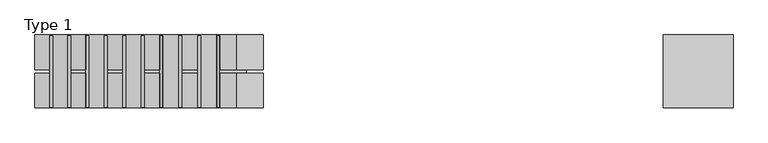
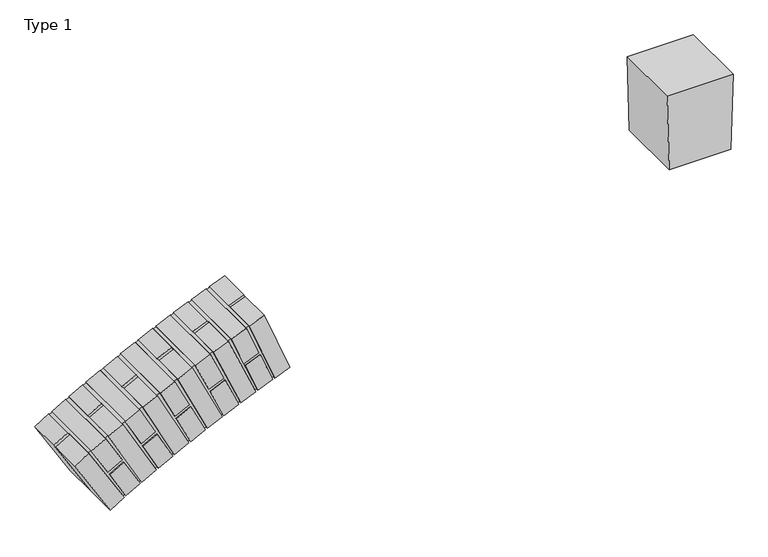
"""IFC4 building model written with IfcOpenShell, lengths in millimetres: proxy geometry, 00_GM_toog : Type 1."""

import ifcopenshell
import ifcopenshell.guid

model = None  # the IFC model being written
_history = None  # IfcOwnerHistory: only IFC2X3 demands one
_inside = {}  # id of a spatial element -> (the spatial element, [elements in it])
_under = {}  # id of a project, library or spatial element -> (it, [spatial elements below it])
_declared = {}  # id of a project -> (the project, [libraries it declares])
_typed = {}  # id of a type object -> (the type object, [elements of that type])
_made_of = {}  # id of a material, layer set ... -> (it, [elements and type objects made of it])


def new_model(schema):
    """Start an empty IFC model of exactly this schema.

    Asked for "IFC4X3", IfcOpenShell would pick the latest addendum, in which some entities
    have other attributes; the version numbers below select the first issue.
    IFC2X3 requires an IfcOwnerHistory on every rooted entity: one is made here for all.
    """
    global model, _history
    if schema == "IFC4X3":
        model = ifcopenshell.file(schema_version=(4, 3, 0, 0))
    else:
        model = ifcopenshell.file(schema=schema)
    _inside.clear()
    _under.clear()
    _declared.clear()
    _typed.clear()
    _made_of.clear()
    _history = None
    if model.schema == "IFC2X3":
        org = make("IfcOrganization", Name="unknown")
        user = make(
            "IfcPersonAndOrganization",
            ThePerson=make("IfcPerson", FamilyName="unknown"),
            TheOrganization=org,
        )
        app = make(
            "IfcApplication",
            ApplicationDeveloper=org,
            Version="unknown",
            ApplicationFullName="unknown",
            ApplicationIdentifier="unknown",
        )
        _history = make(
            "IfcOwnerHistory",
            OwningUser=user,
            OwningApplication=app,
            ChangeAction="ADDED",
            CreationDate=0,
        )
    return model


def make(cls, **values):
    """One entity of the class cls with the attributes given. An attribute that is None is left unset."""
    return model.create_entity(
        cls, **{name: value for name, value in values.items() if value is not None}
    )


def rooted(cls, **values):
    """An entity with a GlobalId (a new one), such as an element, a storey or a relation."""
    return make(cls, GlobalId=ifcopenshell.guid.new(), OwnerHistory=_history, **values)


def si_unit(unit_type, name, prefix=None):
    """IfcSIUnit, for example si_unit("LENGTHUNIT", "METRE", prefix="MILLI")."""
    return make("IfcSIUnit", UnitType=unit_type, Prefix=prefix, Name=name)


def assignment(units):
    """IfcUnitAssignment: the units of a project."""
    return None if units is None else make("IfcUnitAssignment", Units=units)


def point(xyz):
    """IfcCartesianPoint."""
    return None if xyz is None else make("IfcCartesianPoint", Coordinates=xyz)


def direction(xyz):
    """IfcDirection."""
    return None if xyz is None else make("IfcDirection", DirectionRatios=xyz)


def frame(location, z_axis=None, x_axis=None):
    """IfcAxis2Placement3D, a coordinate frame: its origin and axes. An axis left out is left unset."""
    return make(
        "IfcAxis2Placement3D",
        Location=point(location),
        Axis=direction(z_axis),
        RefDirection=direction(x_axis),
    )


def origin():
    """The frame at (0, 0, 0) with its axes left unset."""
    return frame((0.0, 0.0, 0.0))


def place(relative_to, where):
    """IfcLocalPlacement: puts the frame where relative to a parent placement (None: the world)."""
    return make(
        "IfcLocalPlacement", PlacementRelTo=relative_to, RelativePlacement=where
    )


def context(
    kind, dimensions, precision=None, world=None, true_north=None, identifier=None
):
    """IfcGeometricRepresentationContext, for example the 3D "Model" context."""
    return make(
        "IfcGeometricRepresentationContext",
        ContextIdentifier=identifier,
        ContextType=kind,
        CoordinateSpaceDimension=dimensions,
        Precision=precision,
        WorldCoordinateSystem=world,
        TrueNorth=true_north,
    )


def project(units=None, contexts=None):
    """IfcProject with its units and contexts."""
    return rooted(
        "IfcProject",
        Name="project",
        RepresentationContexts=contexts,
        UnitsInContext=assignment(units),
    )


def spatial(cls, under=None, at=None, **own):
    """A site, building, storey or space (cls), placed at a placement, below another one or the project."""
    s = rooted(cls, ObjectPlacement=at, **own)
    if under is not None:
        _under.setdefault(under.id(), (under, []))[1].append(s)
    return s


def polyline(points):
    """IfcPolyline through the points."""
    return make("IfcPolyline", Points=[point(p) for p in points])


def outline(outer, holes=None, kind="AREA"):
    """IfcArbitraryClosedProfileDef: a profile drawn as a closed curve; with holes, ...WithVoids."""
    if holes is None:
        return make("IfcArbitraryClosedProfileDef", ProfileType=kind, OuterCurve=outer)
    return make(
        "IfcArbitraryProfileDefWithVoids",
        ProfileType=kind,
        OuterCurve=outer,
        InnerCurves=holes,
    )


def extrude(swept, where, along, depth):
    """IfcExtrudedAreaSolid: the profile swept, set in the frame where, extruded along a direction by depth."""
    return make(
        "IfcExtrudedAreaSolid",
        SweptArea=swept,
        Position=where,
        ExtrudedDirection=direction(along),
        Depth=depth,
    )


def shape(context_of_items, identifier, shape_type, items):
    """IfcShapeRepresentation: the items that make up one representation, for example the "Body"."""
    return make(
        "IfcShapeRepresentation",
        ContextOfItems=context_of_items,
        RepresentationIdentifier=identifier,
        RepresentationType=shape_type,
        Items=items,
    )


def source(mapping_origin, context_of_items, identifier, shape_type, items):
    """IfcRepresentationMap: a shape defined once, which mapped items show again and again."""
    return make(
        "IfcRepresentationMap",
        MappingOrigin=mapping_origin,
        MappedRepresentation=shape(context_of_items, identifier, shape_type, items),
    )


def transform(
    local_origin,
    x_axis=None,
    y_axis=None,
    z_axis=None,
    scale=None,
    scale2=None,
    scale3=None,
    uniform=True,
):
    """IfcCartesianTransformationOperator3D, or its non-uniform kind. x_axis, y_axis, z_axis: its Axis1, 2, 3."""
    if uniform:
        return make(
            "IfcCartesianTransformationOperator3D",
            Axis1=direction(x_axis),
            Axis2=direction(y_axis),
            LocalOrigin=point(local_origin),
            Scale=scale,
            Axis3=direction(z_axis),
        )
    return make(
        "IfcCartesianTransformationOperator3DnonUniform",
        Axis1=direction(x_axis),
        Axis2=direction(y_axis),
        LocalOrigin=point(local_origin),
        Scale=scale,
        Axis3=direction(z_axis),
        Scale2=scale2,
        Scale3=scale3,
    )


def mapped(mapping_source, mapping_target):
    """IfcMappedItem: shows the shape of a source again, moved by a transform."""
    return make(
        "IfcMappedItem", MappingSource=mapping_source, MappingTarget=mapping_target
    )


def made_of(thing, what):
    """Note that an element or type object is made of a material, layer set ...; save() writes the relation."""
    if what is not None:
        _made_of.setdefault(what.id(), (what, []))[1].append(thing)
    return thing


def element(
    cls,
    number,
    at=None,
    inside=None,
    cuts=None,
    type_object=None,
    material=None,
    context=None,
    identifier="Body",
    shape_type=None,
    held_by="IfcProductDefinitionShape",
    body=None,
    shapes=None,
    **own,
):
    """One element of the class cls, such as IfcWall. Its Tag is "e" and its number.

    at: its placement. inside: the storey or other place that contains it. cuts: it is an
    opening in that element (IfcRelVoidsElement). A single representation is given by context,
    identifier, shape_type and body (its items); several are given by shapes. held_by: the class
    of the entity that holds the representations. save() writes the other relations.
    """
    e = rooted(cls, Tag="e%d" % number, ObjectPlacement=at, **own)
    if body is not None:
        shapes = [shape(context, identifier, shape_type, body)]
    if shapes is not None:
        e.Representation = make(held_by, Representations=shapes)
    if inside is not None:
        _inside.setdefault(inside.id(), (inside, []))[1].append(e)
    if cuts is not None:
        rooted(
            "IfcRelVoidsElement", RelatingBuildingElement=cuts, RelatedOpeningElement=e
        )
    if type_object is not None:
        _typed.setdefault(type_object.id(), (type_object, []))[1].append(e)
    return made_of(e, material)


def aggregate(whole, parts):
    """IfcRelAggregates: a whole, such as a stair, and the parts it consists of."""
    return rooted("IfcRelAggregates", RelatingObject=whole, RelatedObjects=parts)


def save(model, path):
    """Write the relations noted so far, then the file.

    IfcRelAggregates (storeys below a building ...), IfcRelContainedInSpatialStructure (elements
    in a storey), IfcRelDefinesByType, IfcRelAssociatesMaterial and IfcRelDeclares: one each for
    every whole, place, type object, material and project.
    """
    for whole, parts in _under.values():
        aggregate(whole, parts)
    for where, things in _inside.values():
        rooted(
            "IfcRelContainedInSpatialStructure",
            RelatedElements=things,
            RelatingStructure=where,
        )
    for kind, things in _typed.values():
        rooted("IfcRelDefinesByType", RelatedObjects=things, RelatingType=kind)
    for what, things in _made_of.values():
        rooted("IfcRelAssociatesMaterial", RelatedObjects=things, RelatingMaterial=what)
    for by, libraries in _declared.values():
        rooted("IfcRelDeclares", RelatingContext=by, RelatedDefinitions=libraries)
    model.write(path)


def type_1_fda7a26f(model_context):
    return source(origin(), model_context, "Body", "SweptSolid", [
        extrude(outline(polyline([(210.0, -50.0), (110.0, -50.0), (110.0, 0.0), (210.0, 0.0), (210.0, -50.0)])), frame((-1297.7842293, 0.0, -490.2691324), z_axis=(-0.3718579453562054, 0.0, 0.9282896468643079), x_axis=(0.0, 1.0, 0.0)), (0.0, 0.0, 1.0), 210.0),
        extrude(outline(polyline([(100.0, -50.0), (0.0, -50.0), (0.0, 0.0), (100.0, 0.0), (100.0, -50.0)])), frame((-1297.7842293, 0.0, -490.2691324), z_axis=(-0.3718579453562054, 0.0, 0.9282896468643079), x_axis=(0.0, 1.0, 0.0)), (0.0, 0.0, 1.0), 210.0),
        extrude(outline(polyline([(-321.2933048, -1439.8675863), (-509.0431023, -1357.5533987), (-506.5348544, -1351.8323552), (-419.2972383, -1388.4177845), (-399.9600447, -1342.308426), (-487.6985293, -1305.512944), (-485.1911791, -1299.7939481), (-294.8156345, -1376.0553381), (-298.5063263, -1384.8557583), (-390.7250433, -1346.181371), (-410.0622369, -1392.2907295), (-317.8435199, -1430.9651168), (-321.2933048, -1439.8675863)])), frame((0.0, 2.5, 0.0), z_axis=(0.0, 1.0, 0.0), x_axis=(0.0, 0.0, 1.0)), (0.0, 0.0, 1.0), 205.0),
        extrude(outline(polyline([(0.0, -50.0), (0.0, 0.0), (210.0, 0.0), (210.0, -50.0), (0.0, -50.0)])), frame((-1346.181371, 210.0, -390.7250433), z_axis=(-0.38674387286495593, 0.0, 0.9221871701565875), x_axis=(0.0, -1.0, 0.0)), (0.0, 0.0, 1.0), 100.0),
        extrude(outline(polyline([(0.0, -50.0), (0.0, 0.0), (210.0, 0.0), (210.0, -50.0), (0.0, -50.0)])), frame((-1303.6340387, 210.0, -492.1787617), z_axis=(-0.38674387286495593, 0.0, 0.9221871701565875), x_axis=(0.0, -1.0, 0.0)), (0.0, 0.0, 1.0), 100.0),
        extrude(outline(polyline([(210.0, -50.0), (110.0, -50.0), (110.0, 0.0), (210.0, 0.0), (210.0, -50.0)])), frame((-1401.3386497, 0.0, -533.6974503), z_axis=(-0.40152969904724134, 0.0, 0.9158460027663122), x_axis=(0.0, 1.0, 0.0)), (0.0, 0.0, 1.0), 210.0),
        extrude(outline(polyline([(100.0, -50.0), (0.0, -50.0), (0.0, 0.0), (100.0, 0.0), (100.0, -50.0)])), frame((-1401.3386497, 0.0, -533.6974503), z_axis=(-0.40152969904724134, 0.0, 0.9158460027663122), x_axis=(0.0, 1.0, 0.0)), (0.0, 0.0, 1.0), 210.0),
        extrude(outline(polyline([(-369.3800886, -1548.7846238), (-554.3845512, -1460.4728988), (-551.6935484, -1454.8355101), (-465.678088, -1494.2085449), (-444.8675082, -1448.7451556), (-531.3768203, -1409.1460633), (-528.6867806, -1403.5106923), (-340.8632042, -1485.8572264), (-344.835106, -1494.534357), (-435.7618846, -1452.9131974), (-456.5724644, -1498.3765867), (-365.6456858, -1539.9977463), (-369.3800886, -1548.7846238)])), frame((0.0, 2.5, 0.0), z_axis=(0.0, 1.0, 0.0), x_axis=(0.0, 0.0, 1.0)), (0.0, 0.0, 1.0), 205.0),
        extrude(outline(polyline([(0.0, -50.0), (0.0, 0.0), (210.0, 0.0), (210.0, -50.0), (0.0, -50.0)])), frame((-1452.9131974, 210.0, -435.7618846), z_axis=(-0.4162115968719885, 0.0, 0.9092677859845631), x_axis=(0.0, -1.0, 0.0)), (0.0, 0.0, 1.0), 100.0),
        extrude(outline(polyline([(0.0, -50.0), (0.0, 0.0), (210.0, 0.0), (210.0, -50.0), (0.0, -50.0)])), frame((-1407.1239959, 210.0, -535.7942868), z_axis=(-0.4162115968719885, 0.0, 0.9092677859845631), x_axis=(0.0, -1.0, 0.0)), (0.0, 0.0, 1.0), 100.0),
        extrude(outline(polyline([(210.0, -50.0000001), (110.0, -50.0000001), (110.0, 0.0), (210.0, 0.0), (210.0, -50.0000001)])), frame((-1503.4423241, 0.0, -580.4347636), z_axis=(-0.43078576620803966, 0.0, 0.9024542224581545), x_axis=(0.0, 1.0, 0.0)), (0.0, 0.0, 1.0), 210.0),
        extrude(outline(polyline([(100.0, -50.0000001), (0.0, -50.0000001), (0.0, 0.0), (100.0, 0.0), (100.0, -50.0000001)])), frame((-1503.4423241, 0.0, -580.4347636), z_axis=(-0.43078576620803966, 0.0, 0.9024542224581545), x_axis=(0.0, 1.0, 0.0)), (0.0, 0.0, 1.0), 210.0),
        extrude(outline(polyline([(-420.9459785, -1656.0982709), (-603.0135789, -1561.8804337), (-600.1426072, -1556.3325361), (-515.4383507, -1598.452415), (-493.1759289, -1553.6820612), (-578.366509, -1511.3203539), (-575.4965649, -1505.7744419), (-390.4194022, -1594.1208702), (-394.6684022, -1602.6657283), (-484.2091098, -1558.1408848), (-506.4715315, -1602.9112386), (-416.9308239, -1647.4360821), (-420.9459785, -1656.0982709)])), frame((0.0, 2.5, 0.0), z_axis=(0.0, 1.0, 0.0), x_axis=(0.0, 0.0, 1.0)), (0.0, 0.0, 1.0), 205.0),
        extrude(outline(polyline([(0.0, -50.0), (0.0, 0.0), (210.0, 0.0), (210.0, -50.0), (0.0, -50.0)])), frame((-1558.1408848, 210.0, -484.2091098), z_axis=(-0.4452484348076845, 0.0, 0.8954070757489618), x_axis=(0.0, -1.0, 0.0)), (0.0, 0.0, 1.0), 100.0),
        extrude(outline(polyline([(0.0, -49.9999999), (0.0, 0.0), (210.0, 0.0), (210.0, -49.9999999), (0.0, -49.9999999)])), frame((-1509.1572178, 210.0, -582.7166365), z_axis=(-0.4452484348076845, 0.0, 0.8954070757489618), x_axis=(0.0, -1.0, 0.0)), (0.0, 0.0, 1.0), 100.0),
        extrude(outline(polyline([(210.0, -50.0), (110.0, -50.0), (110.0, 0.0), (210.0, 0.0), (210.0, -50.0)])), frame((-1603.9895489, 0.0, -630.4326871), z_axis=(-0.4595958592830959, 0.0, 0.8881281698774298), x_axis=(0.0, 1.0, 0.0)), (0.0, 0.0, 1.0), 210.0),
        extrude(outline(polyline([(100.0, -50.0), (0.0, -50.0), (0.0, 0.0), (100.0, 0.0), (100.0, -50.0)])), frame((-1603.9895489, 0.0, -630.4326871), z_axis=(-0.4595958592830959, 0.0, 0.8881281698774298), x_axis=(0.0, 1.0, 0.0)), (0.0, 0.0, 1.0), 210.0),
        extrude(outline(polyline([(-475.9375905, -1761.6974301), (-654.879842, -1661.6710206), (-651.8318736, -1656.2183574), (-568.5265115, -1701.0414757), (-544.8352952, -1657.0105063), (-628.6189492, -1611.9300392), (-625.5720717, -1606.4793275), (-443.4329252, -1700.7341889), (-447.9546246, -1709.1379283), (-536.0165635, -1661.7554957), (-559.7077798, -1705.7864651), (-471.6458409, -1753.1688977), (-475.9375905, -1761.6974301)])), frame((0.0, 2.5, 0.0), z_axis=(0.0, 1.0, 0.0), x_axis=(0.0, 0.0, 1.0)), (0.0, 0.0, 1.0), 205.0),
        extrude(outline(polyline([(0.0, -50.0), (0.0, 0.0), (210.0, 0.0), (210.0, -50.0), (0.0, -50.0)])), frame((-1661.7554957, 210.0, -536.0165635), z_axis=(-0.47382432607517866, 0.0, 0.8806193888504856), x_axis=(0.0, -1.0, 0.0)), (0.0, 0.0, 1.0), 100.0),
        extrude(outline(polyline([(0.0, -50.0), (0.0, 0.0), (210.0, 0.0), (210.0, -50.0), (0.0, -50.0)])), frame((-1609.6280737, 210.0, -632.8972341), z_axis=(-0.47382432607517866, 0.0, 0.8806193888504856), x_axis=(0.0, -1.0, 0.0)), (0.0, 0.0, 1.0), 100.0),
        extrude(outline(polyline([(210.0, -50.0), (110.0, -50.0), (110.0, 0.0), (210.0, 0.0), (210.0, -50.0)])), frame((-1702.8762319, 0.0, -683.6394602), z_axis=(-0.4879301524148094, 0.0, 0.8728826761738722), x_axis=(0.0, 1.0, 0.0)), (0.0, 0.0, 1.0), 210.0),
        extrude(outline(polyline([(100.0, -50.0), (0.0, -50.0), (0.0, 0.0), (100.0, 0.0), (100.0, -50.0)])), frame((-1702.8762319, 0.0, -683.6394602), z_axis=(-0.4879301524148094, 0.0, 0.8728826761738722), x_axis=(0.0, 1.0, 0.0)), (0.0, 0.0, 1.0), 210.0),
        extrude(outline(polyline([(-534.2979943, -1865.4727794), (-709.9296455, -1759.7413505), (-706.7078359, -1754.3895668), (-624.8876108, -1801.8695209), (-599.7921264, -1758.6235192), (-682.0821166, -1710.8709622), (-678.86146, -1705.5210939), (-499.8488907, -1805.5868102), (-504.6386083, -1813.8407308), (-591.1306117, -1763.6497621), (-616.2260961, -1806.8957638), (-529.7340926, -1857.0867325), (-534.2979943, -1865.4727794)])), frame((0.0, 2.5, 0.0), z_axis=(0.0, 1.0, 0.0), x_axis=(0.0, 0.0, 1.0)), (0.0, 0.0, 1.0), 205.0),
        extrude(outline(polyline([(0.0, -50.0), (0.0, 0.0), (210.0, 0.0), (210.0, -50.0), (0.0, -50.0)])), frame((-1763.6497621, 210.0, -591.1306117), z_axis=(-0.5019096872759921, 0.0, 0.864920034349139), x_axis=(0.0, -1.0, 0.0)), (0.0, 0.0, 1.0), 100.0),
        extrude(outline(polyline([(0.0, -50.0), (0.0, 0.0), (210.0, 0.0), (210.0, -50.0), (0.0, -50.0)])), frame((-1708.4325505, 210.0, -686.2841298), z_axis=(-0.5019096872759921, 0.0, 0.864920034349139), x_axis=(0.0, -1.0, 0.0)), (0.0, 0.0, 1.0), 100.0),
        extrude(outline(polyline([(210.0, -50.0), (110.0, -50.0), (110.0, 0.0), (210.0, 0.0), (210.0, -50.0)])), frame((-1800.0, 0.0, -740.0), z_axis=(-0.5157593123209204, 0.0, 0.8567335243552988), x_axis=(0.0, 1.0, 0.0)), (0.0, 0.0, 1.0), 210.0),
        extrude(outline(polyline([(100.0, -50.0), (0.0, -50.0), (0.0, 0.0), (100.0, 0.0), (100.0, -50.0)])), frame((-1800.0, 0.0, -740.0), z_axis=(-0.5157593123209204, 0.0, 0.8567335243552988), x_axis=(0.0, 1.0, 0.0)), (0.0, 0.0, 1.0), 210.0),
        extrude(outline(polyline([(0.0, 100.8108108), (0.0, -100.8108108), (-240.0, -94.3243243), (-240.0, 94.3243243), (0.0, 100.8108108)])), frame((0.0, 0.0, 0.0), z_axis=(0.0, 1.0, 0.0), x_axis=(0.0, 0.0, 1.0)), (0.0, 0.0, 1.0), 210.0),
    ])


if __name__ == "__main__":
    model = new_model("IFC4")
    model_context = context("Model", 3, world=origin())
    ifc_project = project(units=[si_unit("LENGTHUNIT", "METRE", prefix="MILLI")], contexts=[model_context])
    site = spatial("IfcSite", under=ifc_project)
    building = spatial("IfcBuilding", under=site)
    placement = place(None, origin())
    type_1_shape = type_1_fda7a26f(model_context)
    element("IfcBuildingElementProxy", 1, Name="00_GM_toog : Type 1", ObjectType="00_GM_toog : Type 1", at=placement, inside=building, context=model_context, shape_type="MappedRepresentation", body=[
        mapped(type_1_shape, transform((0.0, 0.0, 0.0), x_axis=(1.0, 0.0, 0.0), y_axis=(0.0, 1.0, 0.0), z_axis=(0.0, 0.0, 1.0))),
    ])
    save(model, "model.ifc")

# Revit data of these elements
# Type "00_GM_toog : Type 1"
#   straal_hart_rollaag [instance default] = 1935 mm
#   straal_buitenlijn [instance default] = 2040 mm
#   straal [instance default] = 1830 mm
#   stootvoegbreedte_onderzijde [instance default] = 5 mm
#   offset [instance default] = -2070 mm
#   kop_voeg [instance default] = 55 mm
#   hoek_sluitsteen_half [instance default] = 2.80637°
#   hoek_kop [instance default] = 1.72149°
#   halve_breedte_tov_balk [instance default] = 200 mm
#   half_b [instance default] = 1800 mm
#   h_toog [instance default] = 1500 mm
#   h_steen [instance default] = 210 mm
#   h_sluitsteen [instance default] = 240 mm
#   h_kop [instance default] = 50 mm
#   dekdikte [instance default] = 240 mm
#   breedte [instance default] = 4000 mm
#   b_sluitsteen_bovenzijde [instance default] = 200 mm
#   apothema [instance default] = 330 mm
#   aantal_strekken [instance default] = 14
#   materiaal_voeg [instance default] = none
#   materiaal_strek [instance default] = none
#   materiaal_sluitsteen [instance default] = none
#   materiaal_koppen [instance default] = none
#   Default Elevation = 0
# Element 1 (IfcBuildingElementProxy, "00_GM_toog : Type 1")
#   straal_hart_rollaag = 3595 mm
#   straal_buitenlijn = 3700 mm
#   straal = 3490 mm
#   offset = -3730 mm
#   hoek_sluitsteen_half = 1.54816°
#   hoek_kop = 0.902867°
#   h_toog = 500 mm
#   apothema = 2990 mm
